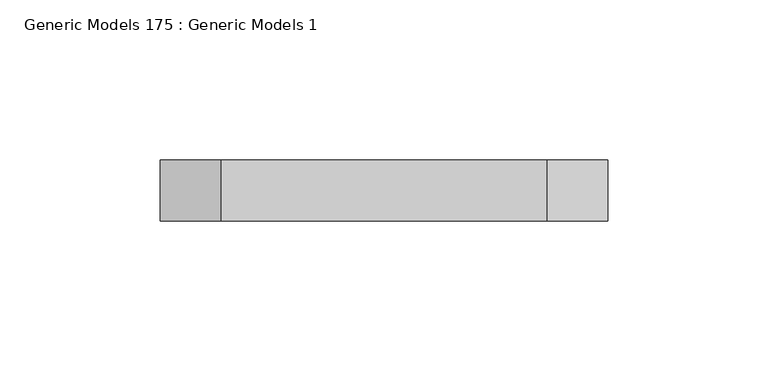
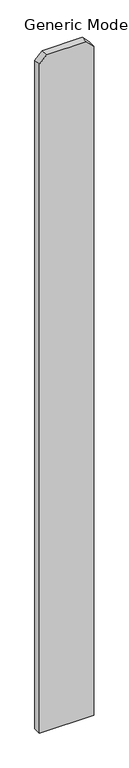
"""IFC4 building model written with IfcOpenShell, lengths in millimetres: proxy geometry, Generic Models 175 : Generic Models 1."""

from ifc_helpers import new_model, si_unit, frame, origin, place, context, project, spatial, polyline, outline, extrude, source, transform, mapped, element, save


def generic_models_175_generic_models_1_480b31b4(model_context):
    return source(origin(), model_context, "Body", "SweptSolid", [
        extrude(outline(polyline([(76.2, -248134.1875), (1885.95, -248134.1875), (1905.0, -248153.2375), (1905.0, -248254.8375), (1885.95, -248273.8875), (76.2, -248273.8875), (76.2, -248134.1875)])), frame((0.0, 547.6875, 0.0), z_axis=(0.0, 1.0, 0.0), x_axis=(0.0, 0.0, 1.0)), (0.0, 0.0, 1.0), 19.05),
    ])


if __name__ == "__main__":
    model = new_model("IFC4")
    model_context = context("Model", 3, world=origin())
    ifc_project = project(units=[si_unit("LENGTHUNIT", "METRE", prefix="MILLI")], contexts=[model_context])
    site = spatial("IfcSite", under=ifc_project)
    building = spatial("IfcBuilding", under=site)
    placement = place(None, origin())
    generic_models_175_generic_models_1_shape = generic_models_175_generic_models_1_480b31b4(model_context)
    element("IfcBuildingElementProxy", 1, Name="Generic Models 175 : Generic Models 1", ObjectType="Generic Models 175 : Generic Models 1", at=placement, inside=building, context=model_context, shape_type="MappedRepresentation", body=[
        mapped(generic_models_175_generic_models_1_shape, transform((0.0, 0.0, 0.0), x_axis=(1.0, 0.0, 0.0), y_axis=(0.0, 1.0, 0.0), z_axis=(0.0, 0.0, 1.0))),
    ])
    save(model, "model.ifc")

# Revit data of these elements
# Element 1 (IfcBuildingElementProxy, "Generic Models 175 : Generic Models 1")
#   Materials on its faces: "VERTICAL 1X6 CEDAR PLANKS W/ CLEAR WOOD SEALER"
# Materials
#   "VERTICAL 1X6 CEDAR PLANKS W/ CLEAR WOOD SEALER": class "Wood", colour RGB 234 198 147, transparency 0, Description = "Pinus Echinata", Cost = 0
